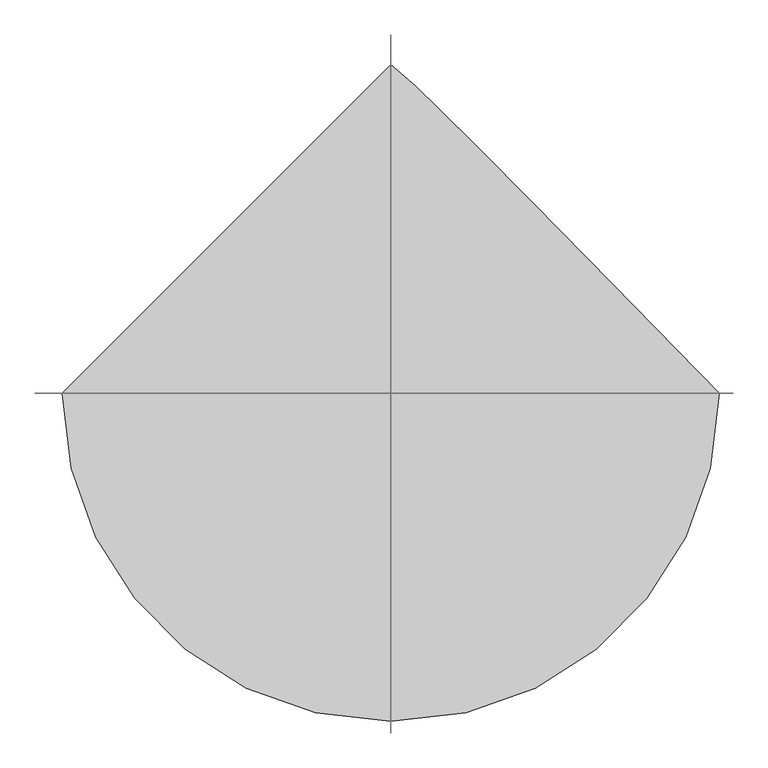
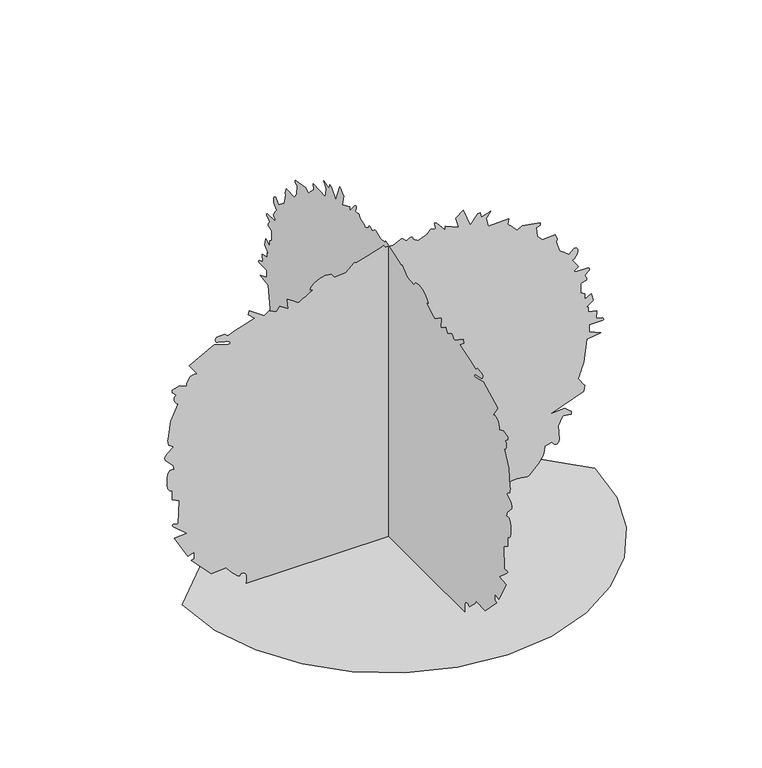
"""IFC4 building model written with IfcOpenShell, lengths in millimetres: proxy geometry, holly 26751 : holly 26751."""

from ifc_helpers import new_model, si_unit, origin, place, context, project, spatial, triangles, source, transform, mapped, element, save


def entourage_54f20335(model_context):
    return source(origin(), model_context, "Body", "Tessellation", [
        triangles([(-823.0310858, 0.0, 7.21e-05), (-801.2709314, -188.5840741, 7.21e-05), (-739.3050917, -361.7670897, 7.21e-05), (-642.0891506, -514.5912643, 7.21e-05), (-514.5912643, -642.0891506, 7.21e-05), (-361.7670897, -739.3050917, 7.21e-05), (-188.5840741, -801.2709314, 7.21e-05), (3.6e-05, -823.0310858, 7.21e-05), (188.5840741, -801.2709314, 7.21e-05), (361.7670897, -739.3050917, 7.21e-05), (514.5912643, -642.0891506, 7.21e-05), (642.0891506, -514.5912643, 7.21e-05), (739.3050917, -361.7670897, 7.21e-05), (801.2709314, -188.5838197, 7.21e-05), (823.0310858, 7.2e-05, 7.21e-05), (555.5640178, 274.3555465, 7.21e-05), (357.2763754, 476.3515926, 7.21e-05), (216.6411551, 618.0454874, 7.21e-05), (122.1254853, 711.5022102, 7.21e-05), (62.2002777, 768.7766939, 7.21e-05), (25.3349997, 801.933827, 7.21e-05), (-0.0001079, 823.0310858, 7.21e-05), (0.0, 364.688096, 1198.1839863), (0.0, 394.9268025, 1235.9816792), (0.0, 406.2653546, 1235.9816792), (0.0, 410.0448841, 1217.0841408), (0.0, 447.8426133, 1228.4226929), (0.0, 428.9450386, 1205.7430452), (0.0, 436.5040612, 1167.9452797), (0.0, 519.6585786, 1171.727389), (0.0, 515.8790491, 1149.0476686), (0.0, 517.7484844, 1147.6176687), (0.0, 521.9039357, 1143.7644882), (0.0, 527.6798913, 1138.1510954), (0.0, 534.4109121, 1131.4328281), (0.0, 541.4314502, 1124.2699659), (0.0, 548.0735593, 1117.3230789), (0.0, 553.6768147, 1111.2499758), (0.0, 572.5743894, 1122.5885279), (0.0, 644.390391, 1111.2499758), (0.0, 644.390391, 1099.9114237), (0.0, 629.2722731, 1096.1318579), (0.0, 633.0517662, 1058.334165), (0.0, 651.9493773, 1035.6544447), (0.0, 704.8677315, 1039.4340105), (0.0, 712.4267904, 1016.7569063), (0.0, 708.6472973, 1009.1953039), (0.0, 719.9858494, 967.6180452), (0.0, 726.0208735, 963.2238367), (0.0, 732.9550432, 957.9761919), (0.0, 740.1179054, 952.4085085), (0.0, 746.8488899, 947.0389961), (0.0, 752.4800869, 942.3932768), (0.0, 756.345912, 938.9998793), (0.0, 757.7835423, 937.3818821), (0.0, 780.4607191, 956.2794931), (0.0, 789.1297394, 953.9172827), (0.0, 793.4883396, 947.7375), (0.0, 794.1741262, 939.096385), (0.0, 791.8195461, 929.3580259), (0.0, 787.0672199, 919.8812788), (0.0, 780.5495945, 912.0225288), (0.0, 772.9016602, 907.1431755), (0.0, 774.118301, 904.8622828), (-2e-07, 781.5884846, 895.1949949), (-2e-07, 794.0852509, 877.4074179), (0.0, 795.5813078, 873.1249758), (0.0, 794.0014624, 870.5621235), (0.0, 782.7695171, 862.2893), (0.0, 780.9686823, 860.2395704), (0.0, 780.4607191, 858.0068579), (2e-07, 785.7515299, 855.1773067), (-2e-07, 836.9528378, 853.0538898), (0.0, 840.9380596, 850.4453281), (1e-07, 841.2580982, 846.6200529), (1e-07, 839.7290491, 843.1504246), (0.0, 822.0405212, 827.768224), (3e-07, 829.193137, 816.4016939), (5e-07, 829.9424372, 812.9472536), (7e-07, 829.5335232, 809.4446331), (7e-07, 829.7087305, 806.8944981), (6e-07, 827.806303, 805.096134), (0.0, 810.7247875, 799.7900625), (0.0, 806.9198599, 797.5295174), (0.0, 806.9198599, 759.7317518), (0.0, 822.0405212, 748.3931997), (0.0, 822.0405212, 725.7135521), (0.0, 848.4971186, 740.8341408), (0.0, 856.0561775, 710.5954342), (0.0, 829.5995075, 691.6952797), (0.0, 837.1585665, 687.9157866), (0.0, 837.1585665, 669.0181755), (0.0, 871.1767662, 661.4591892), (0.0, 867.3972731, 631.2204826), (-4e-07, 892.5458107, 622.5819111), (-3e-07, 895.9697296, 619.724382), (0.0, 897.6334362, 616.1023647), (3e-07, 893.5719835, 613.0467373), (0.0, 840.9380596, 612.3203281), (0.0, 840.9380596, 582.084165), (0.0, 886.2948841, 563.1840105), (0.0, 829.5995075, 555.6249879), (0.0, 818.258412, 461.1319184), (0.0, 815.0631128, 451.4214646), (0.0, 811.202302, 440.3089889), (0.0, 807.0646185, 428.8484965), (0.0, 803.043861, 418.0966819), (0.0, 799.5284506, 409.1101665), (0.0, 796.9122585, 402.9455718), (0.0, 795.5813078, 400.6545053), (0.0, 820.5621958, 364.3553764), (0.0, 822.0405212, 362.856776), (0.0, 818.258412, 340.1796355), (-1.2e-06, 685.9676497, 291.7393147), (0.0, 742.6629536, 294.8203221), (0.0, 767.2044062, 273.0017229), (0.0, 769.1220943, 272.1432179), (0.0, 769.1220943, 260.8046476), (0.0, 735.1038946, 264.5841771), (0.0, 716.2062836, 230.5654505), (6e-07, 720.5065298, 170.5523622), (4e-07, 718.0097345, 161.443416), (0.0, 712.4267904, 154.9702283), (1e-07, 708.1747971, 154.6016643), (1e-07, 704.4080212, 155.6534715), (1e-07, 701.0399855, 157.7794682), (0.0, 689.7471428, 170.0893091), (0.0, 663.2904728, 162.5297596), (0.0, 661.3549805, 143.989803), (0.0, 655.9651205, 127.1831253), (0.0, 637.3164768, 97.7790698), (0.0, 599.0335665, 60.4761278), (0.0, 593.0747369, 58.4339696), (0.0, 555.4065419, 64.3069578), (0.0, 530.3748576, 63.9444981), (0.0, 505.6580887, 55.865013), (0.0, 484.5938948, 35.9298222), (0.0, 470.5222973, 0.0), (1.9e-06, -527.336998, 0.3946068), (1.9e-06, -526.7324927, 3.4093656), (1.8e-06, -525.6326689, 11.1126779), (1.6e-06, -525.1043581, 21.4932261), (1.4e-06, -526.211776, 32.5396858), (1.3e-06, -530.0217905, 42.240454), (1.2e-06, -537.6011244, 48.584103), (1.1e-06, -550.0141022, 49.5597157), (1.1e-06, -552.9884482, 42.5897014), (9e-07, -560.6973527, 44.5830936), (4e-07, -583.0569617, 64.6592528), (2e-07, -594.0755116, 77.3417272), (1e-07, -602.5667084, 88.1867683), (0.0, -606.7119859, 94.4940959), (0.0, -667.1868193, 90.7143212), (0.0, -746.5618435, 173.8690929), (0.0, -735.2232914, 177.6488585), (0.0, -735.2232914, 204.1070183), (0.0, -761.6799614, 196.547487), (0.0, -814.5983156, 291.0408108), (0.0, -765.461998, 294.8203221), (-1e-07, -818.4387789, 340.9873624), (0.0, -822.1573019, 347.7386945), (-3e-07, -820.8568726, 350.2888295), (-4e-07, -818.2406805, 351.2819738), (0.0, -799.4776543, 347.7386945), (0.0, -795.6981611, 442.2317639), (0.0, -822.1573019, 457.352389), (0.0, -822.1573019, 495.1475747), (0.0, -832.8634071, 498.9677267), (1e-07, -839.8280983, 508.9931322), (2e-07, -843.5822296, 523.0672731), (5e-07, -843.58986, 554.7486969), (7e-07, -840.9076109, 568.0481031), (9e-07, -837.1458492, 576.780637), (6e-07, -835.3424709, 579.5238198), (4e-07, -832.4240444, 581.3678933), (1e-07, -824.7836678, 582.9223406), (0.0, -814.5983156, 582.084165), (0.0, -818.9670897, 599.2621862), (0.0, -850.1633686, 632.368523), (0.0, -852.289329, 643.412471), (0.0, -843.1225193, 657.5323214), (0.0, -818.3778088, 676.5772345), (0.0, -819.0966602, 678.065661), (0.0, -834.2578714, 690.2068531), (0.0, -837.2754198, 691.6952797), (0.0, -841.0549129, 714.375), (0.0, -838.9950096, 718.3525915), (0.0, -829.7163609, 789.9704584), (0.0, -799.4776543, 854.2273647), (0.0, -805.1469303, 855.9037886), (0.0, -809.7265926, 860.3360762), (0.0, -812.954884, 866.6098938), (0.0, -814.5627073, 873.8234797), (0.0, -814.2909216, 881.0700577), (0.0, -811.8703571, 887.4378376), (0.0, -807.0392567, 892.0251303), (0.0, -807.4354534, 892.8607624), (0.0, -812.0837162, 897.9737497), (0.0, -820.8492422, 906.3049999), (0.0, -822.1573019, 907.1431755), (0.0, -822.1573019, 918.4817276), (0.0, -791.9185953, 926.0407866), (0.0, -790.6511581, 925.0044399), (0.0, -777.4609749, 918.7560568), (0.0, -765.461998, 914.7022345), (0.0, -764.4104633, 924.481216), (0.0, -761.392915, 934.0036726), (0.0, -756.6100674, 942.5457384), (0.0, -750.2651785, 949.3884893), (0.0, -742.5613609, 953.8080597), (0.0, -733.6992565, 955.0856707), (0.0, -723.8821959, 952.5), (0.0, -754.1209024, 997.8567518), (0.0, -655.8482672, 1050.775106), (7e-07, -598.9294304, 1033.6808733), (5e-07, -592.5108541, 1034.3742903), (5e-07, -591.6802726, 1035.5045992), (4e-07, -591.6421935, 1037.1784796), (3e-07, -592.2771838, 1039.2003038), (2e-07, -595.0864237, 1043.5360857), (0.0, -599.1504198, 1046.9930695), (0.0, -613.793494, 1050.1477461), (0.0, -641.0578909, 1056.558692), (0.0, -644.5071716, 1058.334165), (1e-07, -646.8948166, 1060.1705355), (1e-07, -648.7185425, 1062.5454632), (1e-07, -649.9529875, 1065.3064138), (1e-07, -650.5574564, 1068.3061581), (0.0, -650.5041166, 1071.3923069), (0.0, -649.7573599, 1074.4174129), (0.0, -648.2892809, 1077.2317034), (-2e-07, -645.2513849, 1079.2662449), (0.0, -614.2710085, 1081.0112692), (0.0, -603.3617543, 1070.5744062), (0.0, -602.9299493, 1069.6727171), (0.0, -567.8931707, 1083.2083735), (0.0, -547.3801423, 1090.3508154), (0.0, -493.3187983, 1107.47041), (0.0, -519.7754319, 1130.1475868), (0.0, -515.9959024, 1145.2681755), (0.0, -455.5210327, 1103.6909168), (0.0, -436.6209146, 1118.8089621), (0.0, -406.382208, 1103.6909168), (0.0, -405.4525772, 1104.4097683), (0.0, -396.018996, 1119.5709795), (0.0, -395.0436559, 1122.5885279), (0.0, -361.0254198, 1099.9114237), (0.0, -365.1427557, 1139.9113077), (0.0, -364.8049493, 1141.4886824), (0.0, -342.607903, 1128.2831657), (0.0, -319.4481611, 1111.2499758), (0.0, -309.9866747, 1116.2283783), (0.0, -299.4278897, 1122.1567228), (0.0, -288.7040166, 1128.4457285), (0.0, -278.7446681, 1134.4934698), (0.0, -270.4795113, 1139.7106659), (0.0, -264.8381769, 1143.5003328), (0.0, -262.752839, 1145.2681755), (0.0, -273.3471778, 1149.5912401), (0.0, -269.0418629, 1159.9925674), (0.0, -254.1727123, 1172.6036436), (0.0, -233.0803043, 1183.5662739), (0.0, -210.0991489, 1189.0196474), (0.0, -189.5657729, 1185.1004826), (0.0, -175.8177748, 1167.9452797), (0.0, -130.4607414, 1171.727389), (0.0, -96.4430322, 1201.9634794), (0.0, -95.7204019, 1201.8238077), (0.0, -89.6495515, 1198.8037886), (0.0, -88.8834827, 1198.1839863), (0.0, -39.7464248, 1213.3046476), (0.0, 20.7297008, 1232.2022587), (0.0, 21.3109812, 1231.442712), (0.0, 21.9957141, 1230.3632721), (0.0, 22.7131871, 1229.0906754), (0.0, 23.3937551, 1227.7547104), (0.0, 23.9666262, 1226.4821136), (0.0, 24.3619509, 1225.4026737), (0.0, 24.5094506, 1224.6431271), (0.0, 58.527187, 1220.8637066), (0.0, 88.228163, 1235.3035229), (0.0, 92.5451506, 1235.9816792), (-1e-07, 95.4963785, 1234.686264), (0.0, 109.5573117, 1221.6231079), (0.0, 111.4440243, 1220.8637066), (0.0, 122.4526365, 1227.7801449), (0.0, 128.2821862, 1229.7790054), (0.0, 133.4833494, 1229.5072197), (0.0, 137.0317248, 1225.6972778), (0.0, 137.9024383, 1217.0841408), (0.0, 140.9202138, 1215.7049372), (0.0, 144.3867991, 1213.9269207), (0.0, 147.9687116, 1211.9380886), (0.0, 151.3339586, 1209.9340685), (0.0, 154.1492937, 1208.1052557), (0.0, 156.0827331, 1206.6447344), (0.0, 156.801312, 1205.7430452), (0.0, 162.3971732, 1208.1433348), (0.0, 169.0263289, 1210.9119158), (0.0, 176.0290991, 1213.7770752), (0.0, 182.746894, 1216.4745123), (0.0, 188.5205787, 1218.7325867), (0.0, 192.691, 1220.2871429), (0.0, 194.5987869, 1220.8637066), (0.0, 205.4400219, 1235.8141022), (0.0, 205.9381202, 1235.9816792), (0.0, 208.316318, 1235.3645657), (0.0, 227.1496525, 1232.3444012), (0.0, 228.6167504, 1232.2022587), (1e-07, 223.3642912, 1249.3599323), (1e-07, 222.9002389, 1253.4188416), (1e-07, 223.3033211, 1256.642046), (0.0, 224.8369848, 1258.6613995), (-3e-07, 231.8636453, 1254.2900093), (0.0, 264.139673, 1215.5067661), (0.0, 266.4129717, 1213.3046476), (0.0, 266.4129717, 1228.4226929), (0.0, 319.3313441, 1205.7430452), (0.0, 307.9927557, 1247.3202312), (0.0, 338.2289188, 1269.9999516), (325.0107576, -3.63e-05, 1198.1839863), (355.2494642, -3.85e-05, 1235.9816792), (366.5880163, -3.85e-05, 1235.9816792), (370.3675458, -3.74e-05, 1217.0841408), (408.165275, -3.81e-05, 1228.4226929), (389.2677003, -3.67e-05, 1205.7430452), (396.8267229, -3.44e-05, 1167.9452797), (479.9812403, -3.47e-05, 1171.727389), (476.2017108, -3.33e-05, 1149.0476686), (478.0711461, -3.32e-05, 1147.6176687), (482.2265974, -3.3e-05, 1143.7644882), (488.002553, -3.27e-05, 1138.1510954), (494.7335738, -3.23e-05, 1131.4328281), (501.7515684, -3.18e-05, 1124.2699659), (508.396221, -3.14e-05, 1117.3230789), (513.9994763, -3.11e-05, 1111.2499758), (532.897051, -3.17e-05, 1122.5885279), (604.7130163, -3.11e-05, 1111.2499758), (604.7130163, -3.04e-05, 1099.9114237), (589.5949347, -3.02e-05, 1096.1318579), (593.3744642, -2.79e-05, 1058.334165), (612.2720753, -2.66e-05, 1035.6544447), (665.187886, -2.68e-05, 1039.4340105), (672.7494884, -2.54e-05, 1016.7569063), (668.9699226, -2.5e-05, 1009.1953039), (680.3084747, -2.25e-05, 967.6180452), (686.3434988, -2.22e-05, 963.2238367), (693.2777412, -2.19e-05, 957.9761919), (700.4405308, -2.16e-05, 952.4085085), (707.1715153, -2.13e-05, 947.0389961), (712.8027122, -2.1e-05, 942.3932768), (716.66861, -2.08e-05, 938.9998793), (718.1062403, -2.07e-05, 937.3818821), (740.7833445, -2.18e-05, 956.2794931), (749.4523647, -2.17e-05, 953.9172827), (753.8110376, -2.13e-05, 947.7375), (754.4942808, -2.08e-05, 939.096385), (752.1422441, -2.02e-05, 929.3580259), (747.3899179, -1.97e-05, 919.8812788), (740.8722198, -1.92e-05, 912.0225288), (733.2242855, -1.89e-05, 907.1431755), (734.440999, -1.87e-05, 904.8622828), (741.9111099, -1.8e-05, 895.1949949), (754.4078762, -1.69e-05, 877.4074179), (755.9040058, -1.69e-05, 873.1249758), (754.3240877, -1.68e-05, 870.5621235), (743.0922152, -1.62e-05, 862.2893), (741.2913803, -1.61e-05, 860.2395704), (740.7833445, -1.6e-05, 858.0068579), (746.0741552, -1.6e-05, 855.1773067), (797.2754631, -1.54e-05, 853.0538898), (801.2607576, -1.55e-05, 850.4453281), (801.5807962, -1.54e-05, 846.6200529), (800.0516745, -1.52e-05, 843.1504246), (782.3606031, -1.42e-05, 827.768224), (789.5157623, -1.38e-05, 816.4016939), (790.2650625, -1.38e-05, 812.9472536), (789.8561485, -1.38e-05, 809.4446331), (790.0314285, -1.36e-05, 806.8944981), (788.1289284, -1.34e-05, 805.096134), (771.0474855, -1.25e-05, 799.7900625), (767.2425579, -1.24e-05, 797.5295174), (767.2425579, -1.01e-05, 759.7317518), (782.3606031, -9.4e-06, 748.3931997), (782.3606031, -8.1e-06, 725.7135521), (808.8198166, -9e-06, 740.8341408), (816.3788029, -7.2e-06, 710.5954342), (789.9222055, -6.1e-06, 691.6952797), (797.4812645, -5.8e-06, 687.9157866), (797.4812645, -4.7e-06, 669.0181755), (831.4994642, -4.3e-06, 661.4591892), (827.7198984, -2.5e-06, 631.2204826), (852.8684361, -1.6e-06, 622.5819111), (856.292355, -1.5e-06, 619.724382), (857.9560616, -1.6e-06, 616.1023647), (853.8946089, -1.7e-06, 613.0467373), (801.2607576, -1.3e-06, 612.3203281), (801.2607576, 5e-07, 582.084165), (846.6175095, 1.6e-06, 563.1840105), (789.9222055, 2e-06, 555.6249879), (778.58111, 7.7e-06, 461.1319184), (775.3857382, 8.3e-06, 451.4214646), (771.525, 8.9e-06, 440.3089889), (767.3873165, 9.6e-06, 428.8484965), (763.3664864, 1.02e-05, 418.0966819), (759.8511486, 1.08e-05, 409.1101665), (757.2349566, 1.11e-05, 402.9455718), (755.9040058, 1.13e-05, 400.6545053), (780.8823503, 1.34e-05, 364.3553764), (782.3606031, 1.35e-05, 362.856776), (778.58111, 1.49e-05, 340.1796355), (646.290275, 1.9e-05, 291.7393147), (702.9855789, 1.76e-05, 294.8203221), (727.5271042, 1.89e-05, 273.0017229), (729.4447924, 1.89e-05, 272.1432179), (729.4447924, 1.96e-05, 260.8046476), (695.4265926, 1.94e-05, 264.5841771), (676.5289816, 2.14e-05, 230.5654505), (680.8292278, 2.44e-05, 170.5523622), (678.3323599, 2.51e-05, 161.4436704), (672.7494884, 2.59e-05, 154.9702283), (668.4974951, 2.59e-05, 154.6016643), (664.7306465, 2.58e-05, 155.6534715), (661.3626108, 2.56e-05, 157.7794682), (650.0697681, 2.5e-05, 170.0893091), (623.6106274, 2.55e-05, 162.5297596), (621.675135, 2.66e-05, 143.989803), (616.2852751, 2.76e-05, 127.1833797), (597.6391022, 2.93e-05, 97.7790698), (559.3562282, 3.16e-05, 60.4761278), (553.3948551, 3.17e-05, 58.4342239), (515.7292036, 3.13e-05, 64.3069578), (490.6975193, 3.14e-05, 63.9444981), (465.9807504, 3.18e-05, 55.8652674), (444.9165565, 3.3e-05, 35.9298222), (430.844959, 3.52e-05, 5e-05), (-567.0143363, 3.32e-05, 0.3946575), (-566.409831, 3.31e-05, 3.4094164), (-565.3100072, 3.27e-05, 11.1127279), (-564.7816964, 3.23e-05, 21.4932761), (-565.8891143, 3.18e-05, 32.5396858), (-569.6991288, 3.14e-05, 42.240454), (-577.2784627, 3.11e-05, 48.584103), (-589.6914405, 3.11e-05, 49.5597157), (-592.6657866, 3.16e-05, 42.5897014), (-600.374691, 3.16e-05, 44.5830936), (-622.7343, 3.09e-05, 64.6592528), (-633.7528135, 3.03e-05, 77.3417272), (-642.244083, 2.98e-05, 88.1867683), (-646.3893242, 2.95e-05, 94.4940959), (-706.8641939, 2.98e-05, 90.7143212), (-786.2392181, 2.48e-05, 173.8690929), (-774.900666, 2.46e-05, 177.6488585), (-774.900666, 2.3e-05, 204.1072726), (-801.3598068, 2.35e-05, 196.5477413), (-854.2756176, 1.78e-05, 291.0408108), (-805.1393, 1.76e-05, 294.8203221), (-858.1160809, 1.5e-05, 340.9873624), (-861.8346766, 1.44e-05, 347.7386945), (-860.5341745, 1.46e-05, 350.2888295), (-857.9179825, 1.46e-05, 351.2819738), (-839.1550289, 1.44e-05, 347.7386945), (-835.3754631, 8.8e-06, 442.2317639), (-861.8346766, 7.9e-06, 457.352389), (-861.8346766, 5.7e-06, 495.1475747), (-872.5433252, 5.4e-06, 498.9677267), (-879.5054729, 4.7e-06, 508.9931322), (-883.2595316, 3.8e-06, 523.0672731), (-883.2671619, 1.6e-06, 554.7486969), (-880.5874563, 6e-07, 568.0481031), (-876.8257673, -2e-07, 576.780637), (-875.0197729, 0.0, 579.5238198), (-872.1013464, 1e-07, 581.3678933), (-864.4610424, 3e-07, 582.9223406), (-854.2756176, 5e-07, 582.084165), (-858.6443916, -6e-07, 599.2621862), (-889.8406706, -2.5e-06, 632.368523), (-891.9667036, -3.2e-06, 643.412471), (-882.8023647, -4e-06, 657.5323214), (-858.0551834, -5.2e-06, 676.5772345), (-858.7739622, -5.2e-06, 678.065661), (-873.9352461, -6e-06, 690.2068531), (-876.9527218, -6.1e-06, 691.6952797), (-880.734831, -7.4e-06, 714.375), (-878.6723116, -7.7e-06, 718.3525915), (-869.3937355, -1.19e-05, 789.9704584), (-839.1550289, -1.57e-05, 854.2273647), (-844.824305, -1.58e-05, 855.9037886), (-849.4064381, -1.61e-05, 860.3360762), (-852.6322586, -1.65e-05, 866.6098938), (-854.240082, -1.69e-05, 873.8234797), (-853.9682962, -1.73e-05, 881.0700577), (-851.5476591, -1.77e-05, 887.4378376), (-846.7165586, -1.8e-05, 892.0225868), (-847.1128281, -1.81e-05, 892.8607624), (-851.7610182, -1.84e-05, 897.9737497), (-860.5265442, -1.89e-05, 906.3049999), (-861.8346766, -1.89e-05, 907.1431755), (-861.8346766, -1.96e-05, 918.4817276), (-831.59597, -2e-05, 926.0407866), (-830.3285328, -2e-05, 925.0044399), (-817.1382769, -1.96e-05, 918.7560568), (-805.1393, -1.94e-05, 914.7022345), (-804.0877653, -1.99e-05, 924.481216), (-801.0702169, -2.05e-05, 934.0036726), (-796.287442, -2.1e-05, 942.5457384), (-789.9424805, -2.14e-05, 949.3884893), (-782.2386629, -2.17e-05, 953.8080597), (-773.3766312, -2.18e-05, 955.0856707), (-763.5620413, -2.16e-05, 952.5), (-793.7982044, -2.43e-05, 997.8567518), (-695.5256418, -2.75e-05, 1050.775106), (-638.606805, -2.72e-05, 1033.6808733), (-632.1882288, -2.7e-05, 1034.3742903), (-631.3576109, -2.7e-05, 1035.5045992), (-631.3195318, -2.71e-05, 1037.1784796), (-631.9545221, -2.71e-05, 1039.2003038), (-634.7637257, -2.72e-05, 1043.5360857), (-638.8277218, -2.72e-05, 1046.9930695), (-653.4708687, -2.74e-05, 1050.1477461), (-680.7351929, -2.78e-05, 1056.558692), (-684.1870897, -2.79e-05, 1058.334165), (-686.5721186, -2.81e-05, 1060.1705355), (-688.3983879, -2.83e-05, 1062.5454632), (-689.6302895, -2.84e-05, 1065.3064138), (-690.234831, -2.86e-05, 1068.3061581), (-690.1814913, -2.87e-05, 1071.3923069), (-689.4347345, -2.89e-05, 1074.4174129), (-687.9665829, -2.9e-05, 1077.2317034), (-684.9287596, -2.9e-05, 1079.2637741), (-653.9483831, -2.93e-05, 1081.0112692), (-643.0390926, -2.86e-05, 1070.5744062), (-642.609831, -2.86e-05, 1069.6727171), (-607.5705091, -2.94e-05, 1083.2083735), (-587.0574806, -2.98e-05, 1090.3508154), (-532.9961366, -3.08e-05, 1107.47041), (-559.4527702, -3.22e-05, 1130.1475868), (-555.6732408, -3.31e-05, 1145.2681755), (-495.198371, -3.06e-05, 1103.6909168), (-476.2982529, -3.15e-05, 1118.8089621), (-446.0620897, -3.06e-05, 1103.6909168), (-445.1299155, -3.07e-05, 1104.4097683), (-435.6963344, -3.16e-05, 1119.5709795), (-434.7209942, -3.17e-05, 1122.5885279), (-400.7027581, -3.04e-05, 1099.9114237), (-404.820094, -3.28e-05, 1139.9113077), (-404.484831, -3.29e-05, 1141.4886824), (-382.2852413, -3.21e-05, 1128.2831657), (-359.1254994, -3.11e-05, 1111.2499758), (-349.664013, -3.14e-05, 1116.2283783), (-339.1052098, -3.17e-05, 1122.1567228), (-328.3813368, -3.21e-05, 1128.4457285), (-318.4220246, -3.25e-05, 1134.4934698), (-310.1568315, -3.28e-05, 1139.7106659), (-304.5180405, -3.3e-05, 1143.5003328), (-302.4301774, -3.31e-05, 1145.2681755), (-313.024498, -3.34e-05, 1149.5912401), (-308.7192012, -3.4e-05, 1159.990024), (-293.8500506, -3.47e-05, 1172.6036436), (-272.7578969, -3.54e-05, 1183.5662739), (-249.7767416, -3.57e-05, 1189.0196474), (-229.2433655, -3.55e-05, 1185.1004826), (-215.4953675, -3.44e-05, 1167.9452797), (-170.1383431, -3.47e-05, 1171.727389), (-136.1206249, -3.65e-05, 1201.9634794), (-135.3979945, -3.65e-05, 1201.8238077), (-129.3271442, -3.63e-05, 1198.8037886), (-128.5610754, -3.63e-05, 1198.1839863), (-79.424022, -3.72e-05, 1213.3046476), (-18.9479168, -3.83e-05, 1232.2022587), (-18.3666376, -3.82e-05, 1231.442712), (-17.6819047, -3.82e-05, 1230.3632721), (-16.9644305, -3.81e-05, 1229.0906754), (-16.2838637, -3.8e-05, 1227.7547104), (-15.7109914, -3.79e-05, 1226.4821136), (-15.3156656, -3.79e-05, 1225.4026737), (-15.1681682, -3.78e-05, 1224.6431271), (18.8496693, -3.76e-05, 1220.8637066), (48.5505749, -3.84e-05, 1235.3035229), (52.8675579, -3.85e-05, 1235.9816792), (55.8187858, -3.84e-05, 1234.686264), (69.8797145, -3.76e-05, 1221.6231079), (71.7664271, -3.76e-05, 1220.8637066), (82.7750438, -3.8e-05, 1227.7801449), (88.6045935, -3.81e-05, 1229.7790054), (93.8057568, -3.81e-05, 1229.5072197), (97.3541321, -3.79e-05, 1225.6972778), (98.2248457, -3.74e-05, 1217.0841408), (101.2426211, -3.73e-05, 1215.7049372), (104.7092064, -3.72e-05, 1213.9269207), (108.291119, -3.71e-05, 1211.9380886), (111.6563659, -3.7e-05, 1209.9340685), (114.471701, -3.68e-05, 1208.1052557), (116.4051495, -3.68e-05, 1206.6447344), (117.1234559, -3.67e-05, 1205.7430452), (122.7195896, -3.68e-05, 1208.1433348), (129.3487362, -3.7e-05, 1210.9119158), (136.3515156, -3.72e-05, 1213.7770752), (143.0693014, -3.73e-05, 1216.4745123), (148.8427226, -3.75e-05, 1218.7325867), (153.013153, -3.76e-05, 1220.2871429), (154.9211942, -3.76e-05, 1220.8637066), (165.7624293, -3.85e-05, 1235.8141022), (166.2605275, -3.85e-05, 1235.9816792), (168.6387254, -3.85e-05, 1235.3645657), (187.4720598, -3.83e-05, 1232.3444012), (188.9389034, -3.83e-05, 1232.2022587), (183.6866986, -3.94e-05, 1249.3599323), (183.2226462, -3.96e-05, 1253.4188416), (183.6257285, -3.98e-05, 1256.642046), (185.1593921, -3.99e-05, 1258.6613995), (192.1860526, -3.93e-05, 1254.2900093), (224.4613173, -3.72e-05, 1215.5067661), (226.7366508, -3.72e-05, 1213.3046476), (226.7366508, -3.81e-05, 1228.4226929), (279.6539876, -3.67e-05, 1205.7430452), (268.3128921, -3.92e-05, 1247.3202312), (298.5515805, -4.05e-05, 1269.9999516)], [[21, 22, 1], [20, 21, 1], [19, 20, 1], [18, 19, 1], [17, 18, 1], [17, 1, 2], [17, 2, 3], [17, 3, 4], [16, 17, 4], [16, 4, 5], [16, 5, 6], [16, 6, 7], [16, 7, 8], [16, 8, 9], [16, 9, 10], [16, 10, 11], [16, 11, 12], [15, 16, 12], [14, 15, 12], [13, 14, 12], [100, 101, 102], [26, 27, 28], [153, 154, 155], [157, 158, 159], [316, 317, 318], [239, 240, 241], [238, 239, 241], [319, 320, 23], [318, 319, 23], [245, 246, 247], [87, 88, 89], [156, 157, 159], [29, 30, 31], [138, 139, 140], [248, 249, 250], [138, 140, 141], [117, 118, 119], [116, 117, 119], [212, 213, 214], [138, 141, 142], [258, 259, 260], [312, 313, 314], [311, 312, 314], [310, 311, 314], [92, 93, 94], [138, 142, 143], [146, 147, 148], [39, 40, 41], [39, 41, 42], [24, 25, 26], [96, 97, 98], [200, 201, 202], [199, 200, 202], [198, 199, 202], [198, 202, 203], [197, 198, 203], [44, 45, 46], [44, 46, 47], [309, 310, 314], [258, 260, 261], [197, 203, 204], [196, 197, 204], [137, 138, 143], [271, 272, 273], [271, 273, 274], [271, 274, 275], [271, 275, 276], [271, 276, 277], [271, 277, 278], [271, 278, 279], [95, 96, 98], [94, 95, 98], [94, 98, 99], [92, 94, 99], [247, 248, 250], [137, 143, 144], [23, 24, 26], [241, 242, 243], [87, 89, 90], [247, 250, 251], [115, 116, 119], [115, 119, 120], [114, 115, 120], [90, 91, 92], [112, 113, 114], [111, 112, 114], [110, 111, 114], [165, 166, 167], [39, 42, 43], [38, 39, 43], [244, 245, 247], [160, 161, 162], [160, 162, 163], [160, 163, 164], [55, 56, 57], [55, 57, 58], [55, 58, 59], [55, 59, 60], [55, 60, 61], [55, 61, 62], [55, 62, 63], [184, 185, 186], [85, 86, 87], [266, 267, 268], [266, 268, 269], [266, 269, 270], [73, 74, 75], [73, 75, 76], [72, 73, 76], [72, 76, 77], [66, 67, 68], [80, 81, 82], [44, 47, 48], [159, 160, 164], [23, 26, 28], [23, 28, 29], [153, 155, 156], [66, 68, 69], [212, 214, 215], [65, 66, 69], [258, 261, 262], [122, 123, 124], [122, 124, 125], [122, 125, 126], [121, 122, 126], [121, 126, 127], [287, 288, 289], [287, 289, 290], [286, 287, 290], [285, 286, 290], [179, 180, 181], [179, 181, 182], [178, 179, 182], [136, 137, 144], [243, 244, 247], [65, 69, 70], [184, 186, 187], [183, 184, 187], [196, 204, 205], [152, 153, 156], [136, 144, 145], [263, 264, 265], [262, 263, 265], [258, 262, 265], [120, 121, 127], [114, 120, 127], [114, 127, 128], [146, 148, 149], [167, 168, 169], [167, 169, 170], [79, 80, 82], [78, 79, 82], [78, 82, 83], [77, 78, 83], [72, 77, 83], [72, 83, 84], [71, 72, 84], [309, 314, 315], [305, 306, 307], [304, 305, 307], [281, 282, 283], [280, 281, 283], [280, 283, 284], [64, 65, 70], [152, 156, 159], [167, 170, 171], [167, 171, 172], [167, 172, 173], [167, 173, 174], [167, 174, 175], [167, 175, 176], [167, 176, 177], [165, 167, 177], [159, 164, 165], [304, 307, 308], [230, 231, 232], [229, 230, 232], [228, 229, 232], [227, 228, 232], [226, 227, 232], [225, 226, 232], [224, 225, 232], [223, 224, 232], [223, 232, 233], [222, 223, 233], [222, 233, 234], [222, 234, 235], [221, 222, 235], [220, 221, 235], [220, 235, 236], [219, 220, 236], [218, 219, 236], [218, 236, 237], [217, 218, 237], [217, 237, 238], [132, 133, 134], [131, 132, 134], [189, 190, 191], [189, 191, 192], [189, 192, 193], [189, 193, 194], [189, 194, 195], [189, 195, 196], [189, 196, 205], [183, 187, 188], [212, 215, 216], [152, 159, 165], [130, 131, 134], [129, 130, 134], [128, 129, 134], [128, 134, 135], [114, 128, 135], [114, 135, 136], [114, 136, 145], [110, 114, 145], [109, 110, 145], [108, 109, 145], [107, 108, 145], [106, 107, 145], [105, 106, 145], [104, 105, 145], [103, 104, 145], [102, 103, 145], [100, 102, 145], [99, 100, 145], [92, 99, 145], [90, 92, 145], [87, 90, 145], [85, 87, 145], [84, 85, 145], [71, 84, 145], [70, 71, 145], [64, 70, 145], [63, 64, 145], [55, 63, 145], [54, 55, 145], [53, 54, 145], [52, 53, 145], [51, 52, 145], [50, 51, 145], [49, 50, 145], [48, 49, 145], [44, 48, 145], [43, 44, 145], [38, 43, 145], [37, 38, 145], [36, 37, 145], [35, 36, 145], [34, 35, 145], [33, 34, 145], [32, 33, 145], [31, 32, 145], [29, 31, 145], [23, 29, 145], [318, 23, 145], [316, 318, 145], [315, 316, 145], [309, 315, 145], [308, 309, 145], [304, 308, 145], [303, 304, 145], [302, 303, 145], [301, 302, 145], [300, 301, 145], [299, 300, 145], [298, 299, 145], [297, 298, 145], [296, 297, 145], [295, 296, 145], [294, 295, 145], [293, 294, 145], [292, 293, 145], [291, 292, 145], [290, 291, 145], [285, 290, 145], [284, 285, 145], [280, 284, 145], [279, 280, 145], [271, 279, 145], [270, 271, 145], [266, 270, 145], [265, 266, 145], [258, 265, 145], [257, 258, 145], [256, 257, 145], [255, 256, 145], [254, 255, 145], [253, 254, 145], [252, 253, 145], [251, 252, 145], [247, 251, 145], [243, 247, 145], [241, 243, 145], [241, 145, 146], [241, 146, 149], [241, 149, 150], [241, 150, 151], [241, 151, 152], [241, 152, 165], [241, 165, 177], [241, 177, 178], [241, 178, 182], [238, 241, 182], [217, 238, 182], [216, 217, 182], [212, 216, 182], [212, 182, 183], [212, 183, 188], [212, 188, 189], [212, 189, 205], [212, 205, 206], [212, 206, 207], [212, 207, 208], [212, 208, 209], [211, 212, 209], [210, 211, 209], [398, 399, 400], [324, 325, 326], [451, 452, 453], [455, 456, 457], [614, 615, 616], [537, 538, 539], [536, 537, 539], [617, 618, 321], [616, 617, 321], [543, 544, 545], [385, 386, 387], [454, 455, 457], [327, 328, 329], [436, 437, 438], [546, 547, 548], [436, 438, 439], [415, 416, 417], [414, 415, 417], [510, 511, 512], [436, 439, 440], [556, 557, 558], [610, 611, 612], [609, 610, 612], [608, 609, 612], [390, 391, 392], [436, 440, 441], [444, 445, 446], [337, 338, 339], [337, 339, 340], [322, 323, 324], [394, 395, 396], [498, 499, 500], [497, 498, 500], [496, 497, 500], [496, 500, 501], [495, 496, 501], [342, 343, 344], [342, 344, 345], [607, 608, 612], [556, 558, 559], [495, 501, 502], [494, 495, 502], [435, 436, 441], [569, 570, 571], [569, 571, 572], [569, 572, 573], [569, 573, 574], [569, 574, 575], [569, 575, 576], [569, 576, 577], [393, 394, 396], [392, 393, 396], [392, 396, 397], [390, 392, 397], [545, 546, 548], [435, 441, 442], [321, 322, 324], [539, 540, 541], [385, 387, 388], [545, 548, 549], [413, 414, 417], [413, 417, 418], [412, 413, 418], [388, 389, 390], [410, 411, 412], [409, 410, 412], [408, 409, 412], [463, 464, 465], [337, 340, 341], [336, 337, 341], [542, 543, 545], [458, 459, 460], [458, 460, 461], [458, 461, 462], [353, 354, 355], [353, 355, 356], [353, 356, 357], [353, 357, 358], [353, 358, 359], [353, 359, 360], [353, 360, 361], [482, 483, 484], [383, 384, 385], [564, 565, 566], [564, 566, 567], [564, 567, 568], [371, 372, 373], [371, 373, 374], [370, 371, 374], [370, 374, 375], [364, 365, 366], [378, 379, 380], [342, 345, 346], [457, 458, 462], [321, 324, 326], [321, 326, 327], [451, 453, 454], [364, 366, 367], [510, 512, 513], [363, 364, 367], [556, 559, 560], [420, 421, 422], [420, 422, 423], [420, 423, 424], [419, 420, 424], [419, 424, 425], [585, 586, 587], [585, 587, 588], [584, 585, 588], [583, 584, 588], [477, 478, 479], [477, 479, 480], [476, 477, 480], [434, 435, 442], [541, 542, 545], [363, 367, 368], [482, 484, 485], [481, 482, 485], [494, 502, 503], [450, 451, 454], [434, 442, 443], [561, 562, 563], [560, 561, 563], [556, 560, 563], [418, 419, 425], [412, 418, 425], [412, 425, 426], [444, 446, 447], [465, 466, 467], [465, 467, 468], [377, 378, 380], [376, 377, 380], [376, 380, 381], [375, 376, 381], [370, 375, 381], [370, 381, 382], [369, 370, 382], [607, 612, 613], [603, 604, 605], [602, 603, 605], [579, 580, 581], [578, 579, 581], [578, 581, 582], [362, 363, 368], [450, 454, 457], [465, 468, 469], [465, 469, 470], [465, 470, 471], [465, 471, 472], [465, 472, 473], [465, 473, 474], [465, 474, 475], [463, 465, 475], [457, 462, 463], [602, 605, 606], [528, 529, 530], [527, 528, 530], [526, 527, 530], [525, 526, 530], [524, 525, 530], [523, 524, 530], [522, 523, 530], [521, 522, 530], [521, 530, 531], [520, 521, 531], [520, 531, 532], [520, 532, 533], [519, 520, 533], [518, 519, 533], [518, 533, 534], [517, 518, 534], [516, 517, 534], [516, 534, 535], [515, 516, 535], [515, 535, 536], [430, 431, 432], [429, 430, 432], [487, 488, 489], [487, 489, 490], [487, 490, 491], [487, 491, 492], [487, 492, 493], [487, 493, 494], [487, 494, 503], [481, 485, 486], [510, 513, 514], [450, 457, 463], [428, 429, 432], [427, 428, 432], [426, 427, 432], [426, 432, 433], [412, 426, 433], [412, 433, 434], [412, 434, 443], [408, 412, 443], [407, 408, 443], [406, 407, 443], [405, 406, 443], [404, 405, 443], [403, 404, 443], [402, 403, 443], [401, 402, 443], [400, 401, 443], [398, 400, 443], [397, 398, 443], [390, 397, 443], [388, 390, 443], [385, 388, 443], [383, 385, 443], [382, 383, 443], [369, 382, 443], [368, 369, 443], [362, 368, 443], [361, 362, 443], [353, 361, 443], [352, 353, 443], [351, 352, 443], [350, 351, 443], [349, 350, 443], [348, 349, 443], [347, 348, 443], [346, 347, 443], [342, 346, 443], [341, 342, 443], [336, 341, 443], [335, 336, 443], [334, 335, 443], [333, 334, 443], [332, 333, 443], [331, 332, 443], [330, 331, 443], [329, 330, 443], [327, 329, 443], [321, 327, 443], [616, 321, 443], [614, 616, 443], [613, 614, 443], [607, 613, 443], [606, 607, 443], [602, 606, 443], [601, 602, 443], [600, 601, 443], [599, 600, 443], [598, 599, 443], [597, 598, 443], [596, 597, 443], [595, 596, 443], [594, 595, 443], [593, 594, 443], [592, 593, 443], [591, 592, 443], [590, 591, 443], [589, 590, 443], [588, 589, 443], [583, 588, 443], [582, 583, 443], [578, 582, 443], [577, 578, 443], [569, 577, 443], [568, 569, 443], [564, 568, 443], [563, 564, 443], [556, 563, 443], [555, 556, 443], [554, 555, 443], [553, 554, 443], [552, 553, 443], [551, 552, 443], [550, 551, 443], [549, 550, 443], [545, 549, 443], [541, 545, 443], [539, 541, 443], [539, 443, 444], [539, 444, 447], [539, 447, 448], [539, 448, 449], [539, 449, 450], [539, 450, 463], [539, 463, 475], [539, 475, 476], [539, 476, 480], [536, 539, 480], [515, 536, 480], [514, 515, 480], [510, 514, 480], [510, 480, 481], [510, 481, 486], [510, 486, 487], [510, 487, 503], [510, 503, 504], [510, 504, 505], [510, 505, 506], [510, 506, 507], [509, 510, 507], [508, 509, 507]], closed=False),
    ])


if __name__ == "__main__":
    model = new_model("IFC4")
    model_context = context("Model", 3, world=origin())
    ifc_project = project(units=[si_unit("LENGTHUNIT", "METRE", prefix="MILLI")], contexts=[model_context])
    site = spatial("IfcSite", under=ifc_project)
    building = spatial("IfcBuilding", under=site)
    placement = place(None, origin())
    entourage_shape = entourage_54f20335(model_context)
    element("IfcBuildingElementProxy", 1, Name="holly 26751 : holly 26751", ObjectType="holly 26751 : holly 26751", at=placement, inside=building, context=model_context, shape_type="MappedRepresentation", body=[
        mapped(entourage_shape, transform((0.0, 0.0, 0.0), x_axis=(1.0, 0.0, 0.0), y_axis=(0.0, 1.0, 0.0), z_axis=(0.0, 0.0, 1.0))),
    ])
    save(model, "model.ifc")

# Revit data of these elements
# Type "holly 26751 : holly 26751"
#   built-in parameter 1005195 = "RPC-16-G1GG-0300-7LS3-6000-ST1L-LVER-AU"
#   Height = 0
